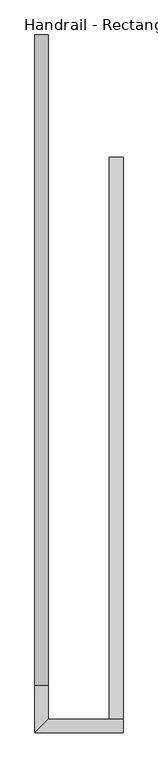
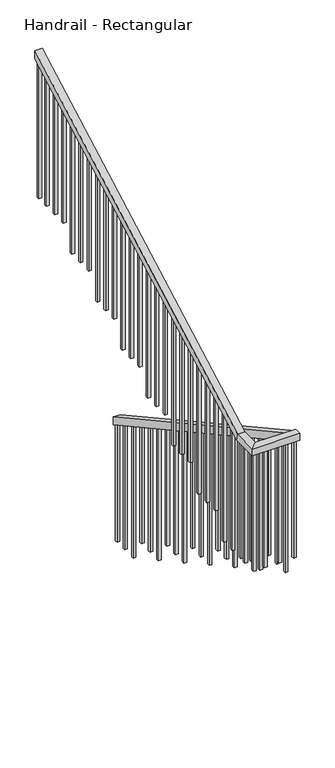
"""IFC4 building model written with IfcOpenShell, lengths in millimetres: railing geometry, Handrail - Rectangular."""

import ifcopenshell
import ifcopenshell.guid

model = None  # the IFC model being written
_history = None  # IfcOwnerHistory: only IFC2X3 demands one
_inside = {}  # id of a spatial element -> (the spatial element, [elements in it])
_under = {}  # id of a project, library or spatial element -> (it, [spatial elements below it])
_declared = {}  # id of a project -> (the project, [libraries it declares])
_typed = {}  # id of a type object -> (the type object, [elements of that type])
_made_of = {}  # id of a material, layer set ... -> (it, [elements and type objects made of it])


def new_model(schema):
    """Start an empty IFC model of exactly this schema.

    Asked for "IFC4X3", IfcOpenShell would pick the latest addendum, in which some entities
    have other attributes; the version numbers below select the first issue.
    IFC2X3 requires an IfcOwnerHistory on every rooted entity: one is made here for all.
    """
    global model, _history
    if schema == "IFC4X3":
        model = ifcopenshell.file(schema_version=(4, 3, 0, 0))
    else:
        model = ifcopenshell.file(schema=schema)
    _inside.clear()
    _under.clear()
    _declared.clear()
    _typed.clear()
    _made_of.clear()
    _history = None
    if model.schema == "IFC2X3":
        org = make("IfcOrganization", Name="unknown")
        user = make(
            "IfcPersonAndOrganization",
            ThePerson=make("IfcPerson", FamilyName="unknown"),
            TheOrganization=org,
        )
        app = make(
            "IfcApplication",
            ApplicationDeveloper=org,
            Version="unknown",
            ApplicationFullName="unknown",
            ApplicationIdentifier="unknown",
        )
        _history = make(
            "IfcOwnerHistory",
            OwningUser=user,
            OwningApplication=app,
            ChangeAction="ADDED",
            CreationDate=0,
        )
    return model


def make(cls, **values):
    """One entity of the class cls with the attributes given. An attribute that is None is left unset."""
    return model.create_entity(
        cls, **{name: value for name, value in values.items() if value is not None}
    )


def rooted(cls, **values):
    """An entity with a GlobalId (a new one), such as an element, a storey or a relation."""
    return make(cls, GlobalId=ifcopenshell.guid.new(), OwnerHistory=_history, **values)


def si_unit(unit_type, name, prefix=None):
    """IfcSIUnit, for example si_unit("LENGTHUNIT", "METRE", prefix="MILLI")."""
    return make("IfcSIUnit", UnitType=unit_type, Prefix=prefix, Name=name)


def assignment(units):
    """IfcUnitAssignment: the units of a project."""
    return None if units is None else make("IfcUnitAssignment", Units=units)


def point(xyz):
    """IfcCartesianPoint."""
    return None if xyz is None else make("IfcCartesianPoint", Coordinates=xyz)


def direction(xyz):
    """IfcDirection."""
    return None if xyz is None else make("IfcDirection", DirectionRatios=xyz)


def frame(location, z_axis=None, x_axis=None):
    """IfcAxis2Placement3D, a coordinate frame: its origin and axes. An axis left out is left unset."""
    return make(
        "IfcAxis2Placement3D",
        Location=point(location),
        Axis=direction(z_axis),
        RefDirection=direction(x_axis),
    )


def origin():
    """The frame at (0, 0, 0) with its axes left unset."""
    return frame((0.0, 0.0, 0.0))


def place(relative_to, where):
    """IfcLocalPlacement: puts the frame where relative to a parent placement (None: the world)."""
    return make(
        "IfcLocalPlacement", PlacementRelTo=relative_to, RelativePlacement=where
    )


def context(
    kind, dimensions, precision=None, world=None, true_north=None, identifier=None
):
    """IfcGeometricRepresentationContext, for example the 3D "Model" context."""
    return make(
        "IfcGeometricRepresentationContext",
        ContextIdentifier=identifier,
        ContextType=kind,
        CoordinateSpaceDimension=dimensions,
        Precision=precision,
        WorldCoordinateSystem=world,
        TrueNorth=true_north,
    )


def project(units=None, contexts=None):
    """IfcProject with its units and contexts."""
    return rooted(
        "IfcProject",
        Name="project",
        RepresentationContexts=contexts,
        UnitsInContext=assignment(units),
    )


def spatial(cls, under=None, at=None, **own):
    """A site, building, storey or space (cls), placed at a placement, below another one or the project."""
    s = rooted(cls, ObjectPlacement=at, **own)
    if under is not None:
        _under.setdefault(under.id(), (under, []))[1].append(s)
    return s


def polyline(points):
    """IfcPolyline through the points."""
    return make("IfcPolyline", Points=[point(p) for p in points])


def outline(outer, holes=None, kind="AREA"):
    """IfcArbitraryClosedProfileDef: a profile drawn as a closed curve; with holes, ...WithVoids."""
    if holes is None:
        return make("IfcArbitraryClosedProfileDef", ProfileType=kind, OuterCurve=outer)
    return make(
        "IfcArbitraryProfileDefWithVoids",
        ProfileType=kind,
        OuterCurve=outer,
        InnerCurves=holes,
    )


def extrude(swept, where, along, depth):
    """IfcExtrudedAreaSolid: the profile swept, set in the frame where, extruded along a direction by depth."""
    return make(
        "IfcExtrudedAreaSolid",
        SweptArea=swept,
        Position=where,
        ExtrudedDirection=direction(along),
        Depth=depth,
    )


def faces_of(points, faces, orient=None, outer=None):
    """IfcFace entities. A face is a list of loops; a loop is a list of indices into points, from 0.

    orient and outer hold one flag for each loop. By default every Orientation is true, the
    first loop of a face is its IfcFaceOuterBound and the others are IfcFaceBound.
    """
    made = []
    for i, loops in enumerate(faces):
        bounds = []
        for j, loop in enumerate(loops):
            is_outer = j == 0 if outer is None else outer[i][j]
            bounds.append(
                make(
                    "IfcFaceOuterBound" if is_outer else "IfcFaceBound",
                    Bound=make("IfcPolyLoop", Polygon=[points[k] for k in loop]),
                    Orientation=True if orient is None else orient[i][j],
                )
            )
        made.append(make("IfcFace", Bounds=bounds))
    return made


def faceted_brep(points, faces, orient=None, outer=None, voids=None):
    """IfcFacetedBrep: a solid bounded by flat faces; with voids (closed shells), ...WithVoids."""
    shared = [point(p) for p in points]
    hull = make("IfcClosedShell", CfsFaces=faces_of(shared, faces, orient, outer))
    if voids is None:
        return make("IfcFacetedBrep", Outer=hull)
    return make(
        "IfcFacetedBrepWithVoids",
        Outer=hull,
        Voids=[
            make(cls, CfsFaces=faces_of(shared, fs, o, b)) for cls, fs, o, b in voids
        ],
    )


def shape(context_of_items, identifier, shape_type, items):
    """IfcShapeRepresentation: the items that make up one representation, for example the "Body"."""
    return make(
        "IfcShapeRepresentation",
        ContextOfItems=context_of_items,
        RepresentationIdentifier=identifier,
        RepresentationType=shape_type,
        Items=items,
    )


def source(mapping_origin, context_of_items, identifier, shape_type, items):
    """IfcRepresentationMap: a shape defined once, which mapped items show again and again."""
    return make(
        "IfcRepresentationMap",
        MappingOrigin=mapping_origin,
        MappedRepresentation=shape(context_of_items, identifier, shape_type, items),
    )


def transform(
    local_origin,
    x_axis=None,
    y_axis=None,
    z_axis=None,
    scale=None,
    scale2=None,
    scale3=None,
    uniform=True,
):
    """IfcCartesianTransformationOperator3D, or its non-uniform kind. x_axis, y_axis, z_axis: its Axis1, 2, 3."""
    if uniform:
        return make(
            "IfcCartesianTransformationOperator3D",
            Axis1=direction(x_axis),
            Axis2=direction(y_axis),
            LocalOrigin=point(local_origin),
            Scale=scale,
            Axis3=direction(z_axis),
        )
    return make(
        "IfcCartesianTransformationOperator3DnonUniform",
        Axis1=direction(x_axis),
        Axis2=direction(y_axis),
        LocalOrigin=point(local_origin),
        Scale=scale,
        Axis3=direction(z_axis),
        Scale2=scale2,
        Scale3=scale3,
    )


def mapped(mapping_source, mapping_target):
    """IfcMappedItem: shows the shape of a source again, moved by a transform."""
    return make(
        "IfcMappedItem", MappingSource=mapping_source, MappingTarget=mapping_target
    )


def made_of(thing, what):
    """Note that an element or type object is made of a material, layer set ...; save() writes the relation."""
    if what is not None:
        _made_of.setdefault(what.id(), (what, []))[1].append(thing)
    return thing


def element(
    cls,
    number,
    at=None,
    inside=None,
    cuts=None,
    type_object=None,
    material=None,
    context=None,
    identifier="Body",
    shape_type=None,
    held_by="IfcProductDefinitionShape",
    body=None,
    shapes=None,
    **own,
):
    """One element of the class cls, such as IfcWall. Its Tag is "e" and its number.

    at: its placement. inside: the storey or other place that contains it. cuts: it is an
    opening in that element (IfcRelVoidsElement). A single representation is given by context,
    identifier, shape_type and body (its items); several are given by shapes. held_by: the class
    of the entity that holds the representations. save() writes the other relations.
    """
    e = rooted(cls, Tag="e%d" % number, ObjectPlacement=at, **own)
    if body is not None:
        shapes = [shape(context, identifier, shape_type, body)]
    if shapes is not None:
        e.Representation = make(held_by, Representations=shapes)
    if inside is not None:
        _inside.setdefault(inside.id(), (inside, []))[1].append(e)
    if cuts is not None:
        rooted(
            "IfcRelVoidsElement", RelatingBuildingElement=cuts, RelatedOpeningElement=e
        )
    if type_object is not None:
        _typed.setdefault(type_object.id(), (type_object, []))[1].append(e)
    return made_of(e, material)


def aggregate(whole, parts):
    """IfcRelAggregates: a whole, such as a stair, and the parts it consists of."""
    return rooted("IfcRelAggregates", RelatingObject=whole, RelatedObjects=parts)


def save(model, path):
    """Write the relations noted so far, then the file.

    IfcRelAggregates (storeys below a building ...), IfcRelContainedInSpatialStructure (elements
    in a storey), IfcRelDefinesByType, IfcRelAssociatesMaterial and IfcRelDeclares: one each for
    every whole, place, type object, material and project.
    """
    for whole, parts in _under.values():
        aggregate(whole, parts)
    for where, things in _inside.values():
        rooted(
            "IfcRelContainedInSpatialStructure",
            RelatedElements=things,
            RelatingStructure=where,
        )
    for kind, things in _typed.values():
        rooted("IfcRelDefinesByType", RelatedObjects=things, RelatingType=kind)
    for what, things in _made_of.values():
        rooted("IfcRelAssociatesMaterial", RelatedObjects=things, RelatingMaterial=what)
    for by, libraries in _declared.values():
        rooted("IfcRelDeclares", RelatingContext=by, RelatedDefinitions=libraries)
    model.write(path)


def handrail_rectangular_2f1847cf(model_context):
    return source(origin(), model_context, "Body", "SolidModel", [
        faceted_brep([(-74523.6, 12185.65, 17490.1411765), (-74472.8, 12185.65, 17490.1411765), (-74472.8, 12185.65, 17432.1885835), (-74523.6, 12185.65, 17432.1885835), (-74523.6, 10077.45, 18647.5843137), (-74523.6, 10077.45, 18589.6317207), (-74472.8, 10077.45, 18589.6317207), (-74472.8, 10077.45, 18647.5843137)], [[[0, 1, 2, 3]], [[4, 5, 6, 7]], [[1, 0, 4, 7]], [[2, 1, 7, 6]], [[3, 2, 6, 5]], [[0, 3, 5, 4]]]),
        faceted_brep([(-74472.8, 10077.45, 18661.5294118), (-74472.8, 10026.65, 18661.5294118), (-74472.8, 10026.65, 18610.7294118), (-74472.8, 10077.45, 18610.7294118), (-74752.2, 10077.45, 18661.5294118), (-74803.0, 10026.65, 18661.5294118), (-74803.0, 10026.65, 18610.7294118), (-74752.2, 10077.45, 18610.7294118), (-74752.2, 10204.45, 18661.5294118), (-74803.0, 10204.45, 18661.5294118), (-74803.0, 10217.4779373, 18610.7294118), (-74752.2, 10217.4779373, 18610.7294118), (-74752.2, 12642.85, 20000.2588235), (-74752.2, 12642.85, 19942.3062305), (-74803.0, 12642.85, 19942.3062305), (-74803.0, 12642.85, 20000.2588235)], [[[0, 1, 2, 3]], [[1, 0, 4, 5]], [[2, 1, 5, 6]], [[3, 2, 6, 7]], [[0, 3, 7, 4]], [[5, 4, 8, 9]], [[6, 5, 9, 10]], [[7, 6, 10, 11]], [[4, 7, 11, 8]], [[12, 13, 14, 15]], [[9, 8, 12, 15]], [[10, 9, 15, 14]], [[11, 10, 14, 13]], [[8, 11, 13, 12]]]),
        extrude(outline(polyline([(12531.725, 19881.2964266), (12550.775, 19891.7552501), (12550.775, 18918.5176471), (12531.725, 18918.5176471), (12531.725, 19881.2964266)])), frame((-74787.125, 0.0, 0.0), z_axis=(1.0, 0.0, 0.0), x_axis=(0.0, 1.0, 0.0)), (0.0, 0.0, 1.0), 19.05),
        extrude(outline(polyline([(12430.125, 19825.5160344), (12449.175, 19835.974858), (12449.175, 18918.5176471), (12430.125, 18918.5176471), (12430.125, 19825.5160344)])), frame((-74787.125, 0.0, 0.0), z_axis=(1.0, 0.0, 0.0), x_axis=(0.0, 1.0, 0.0)), (0.0, 0.0, 1.0), 19.05),
        extrude(outline(polyline([(12328.525, 19769.7356423), (12347.575, 19780.1944658), (12347.575, 18918.5176471), (12328.525, 18918.5176471), (12328.525, 19769.7356423)])), frame((-74787.125, 0.0, 0.0), z_axis=(1.0, 0.0, 0.0), x_axis=(0.0, 1.0, 0.0)), (0.0, 0.0, 1.0), 19.05),
        extrude(outline(polyline([(12226.925, 19713.9552501), (12245.975, 19724.4140737), (12245.975, 18751.1764706), (12226.925, 18751.1764706), (12226.925, 19713.9552501)])), frame((-74787.125, 0.0, 0.0), z_axis=(1.0, 0.0, 0.0), x_axis=(0.0, 1.0, 0.0)), (0.0, 0.0, 1.0), 19.05),
        extrude(outline(polyline([(12125.325, 19658.174858), (12144.375, 19668.6336815), (12144.375, 18751.1764706), (12125.325, 18751.1764706), (12125.325, 19658.174858)])), frame((-74787.125, 0.0, 0.0), z_axis=(1.0, 0.0, 0.0), x_axis=(0.0, 1.0, 0.0)), (0.0, 0.0, 1.0), 19.05),
        extrude(outline(polyline([(12023.725, 19602.3944658), (12042.775, 19612.8532893), (12042.775, 18751.1764706), (12023.725, 18751.1764706), (12023.725, 19602.3944658)])), frame((-74787.125, 0.0, 0.0), z_axis=(1.0, 0.0, 0.0), x_axis=(0.0, 1.0, 0.0)), (0.0, 0.0, 1.0), 19.05),
        extrude(outline(polyline([(11922.125, 19546.6140737), (11941.175, 19557.0728972), (11941.175, 18583.8352941), (11922.125, 18583.8352941), (11922.125, 19546.6140737)])), frame((-74787.125, 0.0, 0.0), z_axis=(1.0, 0.0, 0.0), x_axis=(0.0, 1.0, 0.0)), (0.0, 0.0, 1.0), 19.05),
        extrude(outline(polyline([(11820.525, 19490.8336815), (11839.575, 19501.292505), (11839.575, 18583.8352941), (11820.525, 18583.8352941), (11820.525, 19490.8336815)])), frame((-74787.125, 0.0, 0.0), z_axis=(1.0, 0.0, 0.0), x_axis=(0.0, 1.0, 0.0)), (0.0, 0.0, 1.0), 19.05),
        extrude(outline(polyline([(11718.925, 19435.0532893), (11737.975, 19445.5121129), (11737.975, 18583.8352941), (11718.925, 18583.8352941), (11718.925, 19435.0532893)])), frame((-74787.125, 0.0, 0.0), z_axis=(1.0, 0.0, 0.0), x_axis=(0.0, 1.0, 0.0)), (0.0, 0.0, 1.0), 19.05),
        extrude(outline(polyline([(11617.325, 19379.2728972), (11636.375, 19389.7317207), (11636.375, 18416.4941176), (11617.325, 18416.4941176), (11617.325, 19379.2728972)])), frame((-74787.125, 0.0, 0.0), z_axis=(1.0, 0.0, 0.0), x_axis=(0.0, 1.0, 0.0)), (0.0, 0.0, 1.0), 19.05),
        extrude(outline(polyline([(11515.725, 19323.492505), (11534.775, 19333.9513286), (11534.775, 18416.4941176), (11515.725, 18416.4941176), (11515.725, 19323.492505)])), frame((-74787.125, 0.0, 0.0), z_axis=(1.0, 0.0, 0.0), x_axis=(0.0, 1.0, 0.0)), (0.0, 0.0, 1.0), 19.05),
        extrude(outline(polyline([(11414.125, 19267.7121129), (11433.175, 19278.1709364), (11433.175, 18416.4941176), (11414.125, 18416.4941176), (11414.125, 19267.7121129)])), frame((-74787.125, 0.0, 0.0), z_axis=(1.0, 0.0, 0.0), x_axis=(0.0, 1.0, 0.0)), (0.0, 0.0, 1.0), 19.05),
        extrude(outline(polyline([(11312.525, 19211.9317207), (11331.575, 19222.3905442), (11331.575, 18249.1529412), (11312.525, 18249.1529412), (11312.525, 19211.9317207)])), frame((-74787.125, 0.0, 0.0), z_axis=(1.0, 0.0, 0.0), x_axis=(0.0, 1.0, 0.0)), (0.0, 0.0, 1.0), 19.05),
        extrude(outline(polyline([(11210.925, 19156.1513286), (11229.975, 19166.6101521), (11229.975, 18249.1529412), (11210.925, 18249.1529412), (11210.925, 19156.1513286)])), frame((-74787.125, 0.0, 0.0), z_axis=(1.0, 0.0, 0.0), x_axis=(0.0, 1.0, 0.0)), (0.0, 0.0, 1.0), 19.05),
        extrude(outline(polyline([(11109.325, 19100.3709364), (11128.375, 19110.8297599), (11128.375, 18249.1529412), (11109.325, 18249.1529412), (11109.325, 19100.3709364)])), frame((-74787.125, 0.0, 0.0), z_axis=(1.0, 0.0, 0.0), x_axis=(0.0, 1.0, 0.0)), (0.0, 0.0, 1.0), 19.05),
        extrude(outline(polyline([(11007.725, 19044.5905442), (11026.775, 19055.0493678), (11026.775, 18081.8117647), (11007.725, 18081.8117647), (11007.725, 19044.5905442)])), frame((-74787.125, 0.0, 0.0), z_axis=(1.0, 0.0, 0.0), x_axis=(0.0, 1.0, 0.0)), (0.0, 0.0, 1.0), 19.05),
        extrude(outline(polyline([(10906.125, 18988.8101521), (10925.175, 18999.2689756), (10925.175, 18081.8117647), (10906.125, 18081.8117647), (10906.125, 18988.8101521)])), frame((-74787.125, 0.0, 0.0), z_axis=(1.0, 0.0, 0.0), x_axis=(0.0, 1.0, 0.0)), (0.0, 0.0, 1.0), 19.05),
        extrude(outline(polyline([(10804.525, 18933.0297599), (10823.575, 18943.4885835), (10823.575, 18081.8117647), (10804.525, 18081.8117647), (10804.525, 18933.0297599)])), frame((-74787.125, 0.0, 0.0), z_axis=(1.0, 0.0, 0.0), x_axis=(0.0, 1.0, 0.0)), (0.0, 0.0, 1.0), 19.05),
        extrude(outline(polyline([(10702.925, 18877.2493678), (10721.975, 18887.7081913), (10721.975, 17914.4705882), (10702.925, 17914.4705882), (10702.925, 18877.2493678)])), frame((-74787.125, 0.0, 0.0), z_axis=(1.0, 0.0, 0.0), x_axis=(0.0, 1.0, 0.0)), (0.0, 0.0, 1.0), 19.05),
        extrude(outline(polyline([(10601.325, 18821.4689756), (10620.375, 18831.9277991), (10620.375, 17914.4705882), (10601.325, 17914.4705882), (10601.325, 18821.4689756)])), frame((-74787.125, 0.0, 0.0), z_axis=(1.0, 0.0, 0.0), x_axis=(0.0, 1.0, 0.0)), (0.0, 0.0, 1.0), 19.05),
        extrude(outline(polyline([(10499.725, 18765.6885835), (10518.775, 18776.147407), (10518.775, 17914.4705882), (10499.725, 17914.4705882), (10499.725, 18765.6885835)])), frame((-74787.125, 0.0, 0.0), z_axis=(1.0, 0.0, 0.0), x_axis=(0.0, 1.0, 0.0)), (0.0, 0.0, 1.0), 19.05),
        extrude(outline(polyline([(10398.125, 18709.9081913), (10417.175, 18720.3670148), (10417.175, 17747.1294118), (10398.125, 17747.1294118), (10398.125, 18709.9081913)])), frame((-74787.125, 0.0, 0.0), z_axis=(1.0, 0.0, 0.0), x_axis=(0.0, 1.0, 0.0)), (0.0, 0.0, 1.0), 19.05),
        extrude(outline(polyline([(10296.525, 18654.1277991), (10315.575, 18664.5866227), (10315.575, 17747.1294118), (10296.525, 17747.1294118), (10296.525, 18654.1277991)])), frame((-74787.125, 0.0, 0.0), z_axis=(1.0, 0.0, 0.0), x_axis=(0.0, 1.0, 0.0)), (0.0, 0.0, 1.0), 19.05),
        extrude(outline(polyline([(-74768.075, 10144.125), (-74787.125, 10144.125), (-74787.125, 10163.175), (-74768.075, 10163.175), (-74768.075, 10144.125)])), frame((0.0, 0.0, 17747.1294118), z_axis=(0.0, 0.0, 1.0), x_axis=(1.0, 0.0, 0.0)), (0.0, 0.0, 1.0), 863.6),
        extrude(outline(polyline([(-74691.875, 10061.575), (-74691.875, 10042.525), (-74710.925, 10042.525), (-74710.925, 10061.575), (-74691.875, 10061.575)])), frame((0.0, 0.0, 17747.1294118), z_axis=(0.0, 0.0, 1.0), x_axis=(1.0, 0.0, 0.0)), (0.0, 0.0, 1.0), 863.6),
        extrude(outline(polyline([(-74590.275, 10061.575), (-74590.275, 10042.525), (-74609.325, 10042.525), (-74609.325, 10061.575), (-74590.275, 10061.575)])), frame((0.0, 0.0, 17747.1294118), z_axis=(0.0, 0.0, 1.0), x_axis=(1.0, 0.0, 0.0)), (0.0, 0.0, 1.0), 863.6),
        extrude(outline(polyline([(10144.125, 18553.0258384), (10163.175, 18542.5670148), (10163.175, 17579.7882353), (10144.125, 17579.7882353), (10144.125, 18553.0258384)])), frame((-74507.725, 0.0, 0.0), z_axis=(1.0, 0.0, 0.0), x_axis=(0.0, 1.0, 0.0)), (0.0, 0.0, 1.0), 19.05),
        extrude(outline(polyline([(10245.725, 18497.2454462), (10264.775, 18486.7866227), (10264.775, 17579.7882353), (10245.725, 17579.7882353), (10245.725, 18497.2454462)])), frame((-74507.725, 0.0, 0.0), z_axis=(1.0, 0.0, 0.0), x_axis=(0.0, 1.0, 0.0)), (0.0, 0.0, 1.0), 19.05),
        extrude(outline(polyline([(10347.325, 18441.465054), (10366.375, 18431.0062305), (10366.375, 17579.7882353), (10347.325, 17579.7882353), (10347.325, 18441.465054)])), frame((-74507.725, 0.0, 0.0), z_axis=(1.0, 0.0, 0.0), x_axis=(0.0, 1.0, 0.0)), (0.0, 0.0, 1.0), 19.05),
        extrude(outline(polyline([(10448.925, 18385.6846619), (10467.975, 18375.2258384), (10467.975, 17412.4470588), (10448.925, 17412.4470588), (10448.925, 18385.6846619)])), frame((-74507.725, 0.0, 0.0), z_axis=(1.0, 0.0, 0.0), x_axis=(0.0, 1.0, 0.0)), (0.0, 0.0, 1.0), 19.05),
        extrude(outline(polyline([(10550.525, 18329.9042697), (10569.575, 18319.4454462), (10569.575, 17412.4470588), (10550.525, 17412.4470588), (10550.525, 18329.9042697)])), frame((-74507.725, 0.0, 0.0), z_axis=(1.0, 0.0, 0.0), x_axis=(0.0, 1.0, 0.0)), (0.0, 0.0, 1.0), 19.05),
        extrude(outline(polyline([(10652.125, 18274.1238776), (10671.175, 18263.665054), (10671.175, 17412.4470588), (10652.125, 17412.4470588), (10652.125, 18274.1238776)])), frame((-74507.725, 0.0, 0.0), z_axis=(1.0, 0.0, 0.0), x_axis=(0.0, 1.0, 0.0)), (0.0, 0.0, 1.0), 19.05),
        extrude(outline(polyline([(10753.725, 18218.3434854), (10772.775, 18207.8846619), (10772.775, 17245.1058824), (10753.725, 17245.1058824), (10753.725, 18218.3434854)])), frame((-74507.725, 0.0, 0.0), z_axis=(1.0, 0.0, 0.0), x_axis=(0.0, 1.0, 0.0)), (0.0, 0.0, 1.0), 19.05),
        extrude(outline(polyline([(10855.325, 18162.5630933), (10874.375, 18152.1042697), (10874.375, 17245.1058824), (10855.325, 17245.1058824), (10855.325, 18162.5630933)])), frame((-74507.725, 0.0, 0.0), z_axis=(1.0, 0.0, 0.0), x_axis=(0.0, 1.0, 0.0)), (0.0, 0.0, 1.0), 19.05),
        extrude(outline(polyline([(10956.925, 18106.7827011), (10975.975, 18096.3238776), (10975.975, 17245.1058824), (10956.925, 17245.1058824), (10956.925, 18106.7827011)])), frame((-74507.725, 0.0, 0.0), z_axis=(1.0, 0.0, 0.0), x_axis=(0.0, 1.0, 0.0)), (0.0, 0.0, 1.0), 19.05),
        extrude(outline(polyline([(11058.525, 18051.0023089), (11077.575, 18040.5434854), (11077.575, 17077.7647059), (11058.525, 17077.7647059), (11058.525, 18051.0023089)])), frame((-74507.725, 0.0, 0.0), z_axis=(1.0, 0.0, 0.0), x_axis=(0.0, 1.0, 0.0)), (0.0, 0.0, 1.0), 19.05),
        extrude(outline(polyline([(11160.125, 17995.2219168), (11179.175, 17984.7630933), (11179.175, 17077.7647059), (11160.125, 17077.7647059), (11160.125, 17995.2219168)])), frame((-74507.725, 0.0, 0.0), z_axis=(1.0, 0.0, 0.0), x_axis=(0.0, 1.0, 0.0)), (0.0, 0.0, 1.0), 19.05),
        extrude(outline(polyline([(11261.725, 17939.4415246), (11280.775, 17928.9827011), (11280.775, 17077.7647059), (11261.725, 17077.7647059), (11261.725, 17939.4415246)])), frame((-74507.725, 0.0, 0.0), z_axis=(1.0, 0.0, 0.0), x_axis=(0.0, 1.0, 0.0)), (0.0, 0.0, 1.0), 19.05),
        extrude(outline(polyline([(11363.325, 17883.6611325), (11382.375, 17873.2023089), (11382.375, 16910.4235294), (11363.325, 16910.4235294), (11363.325, 17883.6611325)])), frame((-74507.725, 0.0, 0.0), z_axis=(1.0, 0.0, 0.0), x_axis=(0.0, 1.0, 0.0)), (0.0, 0.0, 1.0), 19.05),
        extrude(outline(polyline([(11464.925, 17827.8807403), (11483.975, 17817.4219168), (11483.975, 16910.4235294), (11464.925, 16910.4235294), (11464.925, 17827.8807403)])), frame((-74507.725, 0.0, 0.0), z_axis=(1.0, 0.0, 0.0), x_axis=(0.0, 1.0, 0.0)), (0.0, 0.0, 1.0), 19.05),
        extrude(outline(polyline([(11566.525, 17772.1003482), (11585.575, 17761.6415246), (11585.575, 16910.4235294), (11566.525, 16910.4235294), (11566.525, 17772.1003482)])), frame((-74507.725, 0.0, 0.0), z_axis=(1.0, 0.0, 0.0), x_axis=(0.0, 1.0, 0.0)), (0.0, 0.0, 1.0), 19.05),
        extrude(outline(polyline([(11668.125, 17716.319956), (11687.175, 17705.8611325), (11687.175, 16743.0823529), (11668.125, 16743.0823529), (11668.125, 17716.319956)])), frame((-74507.725, 0.0, 0.0), z_axis=(1.0, 0.0, 0.0), x_axis=(0.0, 1.0, 0.0)), (0.0, 0.0, 1.0), 19.05),
        extrude(outline(polyline([(11769.725, 17660.5395638), (11788.775, 17650.0807403), (11788.775, 16743.0823529), (11769.725, 16743.0823529), (11769.725, 17660.5395638)])), frame((-74507.725, 0.0, 0.0), z_axis=(1.0, 0.0, 0.0), x_axis=(0.0, 1.0, 0.0)), (0.0, 0.0, 1.0), 19.05),
        extrude(outline(polyline([(11871.325, 17604.7591717), (11890.375, 17594.3003482), (11890.375, 16743.0823529), (11871.325, 16743.0823529), (11871.325, 17604.7591717)])), frame((-74507.725, 0.0, 0.0), z_axis=(1.0, 0.0, 0.0), x_axis=(0.0, 1.0, 0.0)), (0.0, 0.0, 1.0), 19.05),
        extrude(outline(polyline([(11972.925, 17548.9787795), (11991.975, 17538.519956), (11991.975, 16575.7411765), (11972.925, 16575.7411765), (11972.925, 17548.9787795)])), frame((-74507.725, 0.0, 0.0), z_axis=(1.0, 0.0, 0.0), x_axis=(0.0, 1.0, 0.0)), (0.0, 0.0, 1.0), 19.05),
        extrude(outline(polyline([(12074.525, 17493.1983874), (12093.575, 17482.7395638), (12093.575, 16575.7411765), (12074.525, 16575.7411765), (12074.525, 17493.1983874)])), frame((-74507.725, 0.0, 0.0), z_axis=(1.0, 0.0, 0.0), x_axis=(0.0, 1.0, 0.0)), (0.0, 0.0, 1.0), 19.05),
        extrude(outline(polyline([(-74768.075, 10194.925), (-74787.125, 10194.925), (-74787.125, 10213.975), (-74768.075, 10213.975), (-74768.075, 10194.925)])), frame((0.0, 0.0, 17747.1294118), z_axis=(0.0, 0.0, 1.0), x_axis=(1.0, 0.0, 0.0)), (0.0, 0.0, 1.0), 863.6),
        extrude(outline(polyline([(-74768.075, 10061.575), (-74768.075, 10042.525), (-74787.125, 10042.525), (-74787.125, 10061.575), (-74768.075, 10061.575)])), frame((0.0, 0.0, 17747.1294118), z_axis=(0.0, 0.0, 1.0), x_axis=(1.0, 0.0, 0.0)), (0.0, 0.0, 1.0), 863.6),
        extrude(outline(polyline([(10042.525, 18608.8062305), (10061.575, 18598.347407), (10061.575, 17747.1294118), (10042.525, 17747.1294118), (10042.525, 18608.8062305)])), frame((-74507.725, 0.0, 0.0), z_axis=(1.0, 0.0, 0.0), x_axis=(0.0, 1.0, 0.0)), (0.0, 0.0, 1.0), 19.05),
        extrude(outline(polyline([(12623.8, 19931.847407), (12642.85, 19942.3062305), (12642.85, 18918.5176471), (12623.8, 18918.5176471), (12623.8, 19931.847407)])), frame((-74787.125, 0.0, 0.0), z_axis=(1.0, 0.0, 0.0), x_axis=(0.0, 1.0, 0.0)), (0.0, 0.0, 1.0), 19.05),
        extrude(outline(polyline([(12166.6, 17442.647407), (12185.65, 17432.1885835), (12185.65, 16575.7411765), (12166.6, 16575.7411765), (12166.6, 17442.647407)])), frame((-74507.725, 0.0, 0.0), z_axis=(1.0, 0.0, 0.0), x_axis=(0.0, 1.0, 0.0)), (0.0, 0.0, 1.0), 19.05),
    ])


if __name__ == "__main__":
    model = new_model("IFC4")
    model_context = context("Model", 3, world=origin())
    ifc_project = project(units=[si_unit("LENGTHUNIT", "METRE", prefix="MILLI")], contexts=[model_context])
    site = spatial("IfcSite", under=ifc_project)
    building = spatial("IfcBuilding", under=site)
    placement = place(None, origin())
    handrail_rectangular_shape = handrail_rectangular_2f1847cf(model_context)
    element("IfcRailing", 1, ObjectType="Handrail - Rectangular", at=placement, inside=building, context=model_context, shape_type="MappedRepresentation", body=[
        mapped(handrail_rectangular_shape, transform((0.0, 0.0, 0.0), x_axis=(1.0, 0.0, 0.0), y_axis=(0.0, 1.0, 0.0), z_axis=(0.0, 0.0, 1.0))),
    ])
    save(model, "model.ifc")
